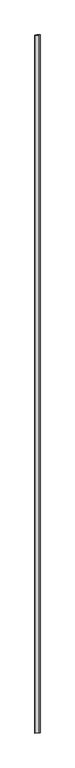
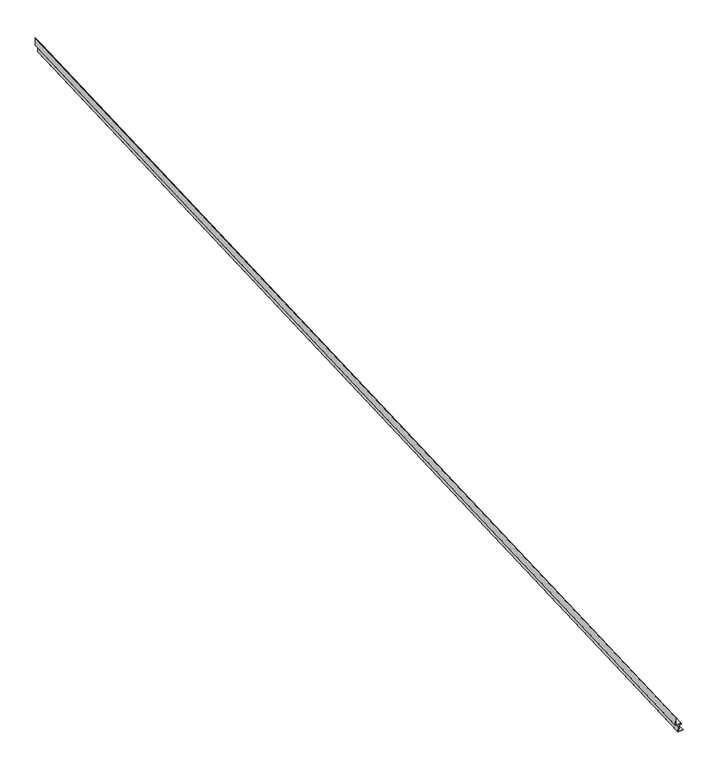
"""IFC4 building model written with IfcOpenShell, lengths in millimetres: proxy geometry, Generic Models 2:Generic Models 2:310765:Generic Models 2:310765 : Generic Models 2:Generic Models 2:310765:199 : Generic Models 2:Generic Models 2:310765:Generic Models 2:310765 : Generic Models 2:Generic Models 2:310765:300385."""

from ifc_helpers import new_model, si_unit, frame, origin, place, context, project, spatial, polyline, outline, extrude, source, transform, mapped, element, save


def generic_models_51ba82ec(model_context):
    return source(origin(), model_context, "Body", "SweptSolid", [
        extrude(outline(polyline([(146.05, 0.0), (146.05, -64.157564), (155.575, -64.157564), (155.575, -46.695064), (157.1625, -46.695064), (157.1625, -65.745064), (144.4624999, -65.745064), (144.4624999, -1.5875), (55.5624999, -1.5875), (55.5624999, 0.0), (146.05, 0.0)])), frame((579355.3367239, -579093.8941479, 4188.3187126), z_axis=(0.0, 0.9991330730923567, 0.041630544712067834), x_axis=(0.0, 0.041630544712067834, -0.9991330730923567)), (0.0, 0.0, 1.0), 12411.242059),
        extrude(outline(polyline([(151.6062499, -42.3509311), (151.6062499, -61.2200628), (150.01875, -61.2200628), (150.01875, -40.7634311), (202.4062499, -40.7634311), (202.4062499, -42.3509311), (151.6062499, -42.3509311)])), frame((579355.3367239, -579093.8941479, 4188.3187126), z_axis=(0.0, 0.9991330730923567, 0.041630544712067834), x_axis=(0.0, 0.041630544712067834, -0.9991330730923567)), (0.0, 0.0, 1.0), 12411.242059),
        extrude(outline(polyline([(235.74375, -30.1625), (235.74375, -91.3825628), (234.15625, -91.3825628), (234.15625, -31.75), (172.2437499, -31.75), (172.2437499, -30.1625), (235.74375, -30.1625)])), frame((579355.3367239, -579093.8941479, 4188.3187126), z_axis=(0.0, 0.9991330730923567, 0.041630544712067834), x_axis=(0.0, 0.041630544712067834, -0.9991330730923567)), (0.0, 0.0, 1.0), 12411.242059),
    ])


if __name__ == "__main__":
    model = new_model("IFC4")
    model_context = context("Model", 3, world=origin())
    ifc_project = project(units=[si_unit("LENGTHUNIT", "METRE", prefix="MILLI")], contexts=[model_context])
    site = spatial("IfcSite", under=ifc_project)
    building = spatial("IfcBuilding", under=site)
    placement = place(None, origin())
    generic_models_shape = generic_models_51ba82ec(model_context)
    element("IfcBuildingElementProxy", 1, Name="Generic Models 2:Generic Models 2:310765:Generic Models 2:310765 : Generic Models 2:Generic Models 2:310765:199 : Generic Models 2:Generic Models 2:310765:Generic Models 2:310765 : Generic Models 2:Generic Models 2:310765:300385", ObjectType="Generic Models 2:Generic Models 2:310765:Generic Models 2:310765 : Generic Models 2:Generic Models 2:310765:199 : Generic Models 2:Generic Models 2:310765:Generic Models 2:310765 : Generic Models 2:Generic Models 2:310765:300385", at=placement, inside=building, context=model_context, shape_type="MappedRepresentation", body=[
        mapped(generic_models_shape, transform((0.0, 0.0, 0.0), x_axis=(1.0, 0.0, 0.0), y_axis=(0.0, 1.0, 0.0), z_axis=(0.0, 0.0, 1.0))),
    ])
    save(model, "model.ifc")

# Revit data of these elements
# Type "Generic Models 2:Generic Models 2:310765:Generic Models 2:310765 : Generic Models 2:Generic Models 2:310765:199 : Generic Models 2:Generic Models 2:310765:Generic Models 2:310765 : Generic Models 2:Generic Models 2:310765:300385"
#   NameOverride = "Generic Models 2:Generic Models 2:310765:Generic Models 2:310765 : Generic Models 2:Generic Models 2:310765:300385"
#   ObjectTypeOverride = "Generic Models 2:310765 : Generic Models 2:Generic Models 2:310765"
#   Reference = "Generic Models 2"
#   Tag = "300385"
# Element 1 (IfcBuildingElementProxy, "Generic Models 2:Generic Models 2:310765:Generic Models 2:310765 : Generic Models 2:Generic Models 2:310765:199 : Generic Models 2:Generic Models 2:310765:Generic Models 2:310765 : Generic Models 2:Generic Models 2:310765:300385")
#   Materials on its faces: "BRAKE METAL FLASHING"
# Materials
#   "BRAKE METAL FLASHING": class "Unassigned", colour RGB 210 209 208, transparency 0, Cost = 0
